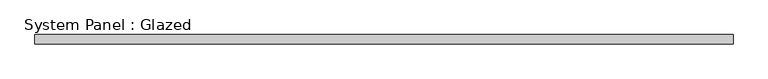
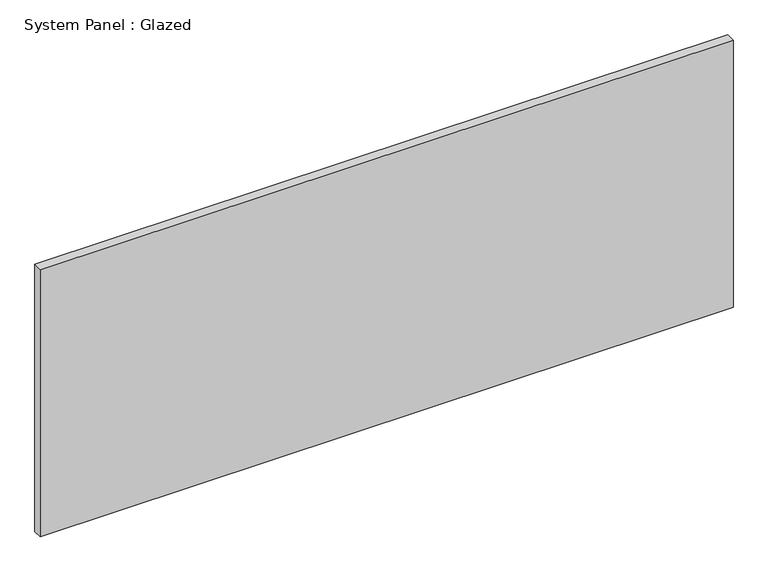
"""IFC4 building model written with IfcOpenShell, lengths in millimetres: plate geometry, System Panel : Glazed."""

from ifc_helpers import new_model, si_unit, origin, origin_with_axes, place, context, project, spatial, polyline, outline, extrude, source, transform, mapped, element, save


def system_panel_glazed_08779d50(model_context):
    return source(origin(), model_context, "Body", "SweptSolid", [
        extrude(outline(polyline([(949.9999998, 24.5), (-949.9999998, 24.5), (-949.9999998, 49.5), (949.9999998, 49.5), (949.9999998, 24.5)])), origin_with_axes(), (0.0, 0.0, 1.0), 775.0),
    ])


if __name__ == "__main__":
    model = new_model("IFC4")
    model_context = context("Model", 3, world=origin())
    ifc_project = project(units=[si_unit("LENGTHUNIT", "METRE", prefix="MILLI")], contexts=[model_context])
    site = spatial("IfcSite", under=ifc_project)
    building = spatial("IfcBuilding", under=site)
    placement = place(None, origin())
    system_panel_glazed_shape = system_panel_glazed_08779d50(model_context)
    element("IfcPlate", 1, ObjectType="System Panel : Glazed", at=placement, inside=building, context=model_context, shape_type="MappedRepresentation", body=[
        mapped(system_panel_glazed_shape, transform((0.0, 0.0, 0.0), x_axis=(1.0, 0.0, 0.0), y_axis=(0.0, 1.0, 0.0), z_axis=(0.0, 0.0, 1.0))),
    ])
    save(model, "model.ifc")

# Revit data of these elements
# Element 1 (IfcPlate, "System Panel : Glazed")
#   Materials on its faces: "Glass"
# Materials
#   "Glass": class "Glass", colour RGB 0 128 192, transparency 0.9
